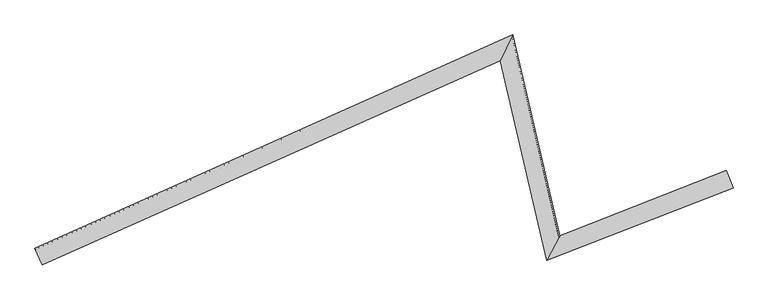
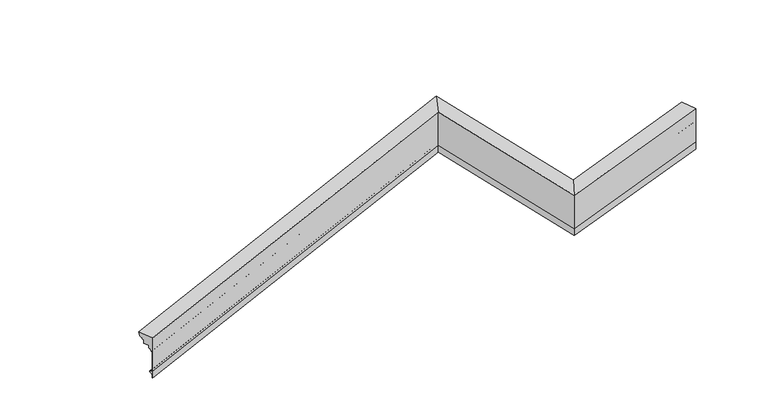
"""IFC4 building model written with IfcOpenShell, lengths in millimetres: proxy geometry, 41_GMA_lijst_1 : 41_GMA_lijst_1."""

from ifc_helpers import new_model, si_unit, frame, origin, place, context, project, spatial, polyline, circle_curve, ellipse_curve, source, transform, mapped, element, save
from ifc_brep_helpers import plane_surface, cylinder_surface, revolved_surface, advanced_brep


def generic_models_faa5d878(model_context):
    return source(origin(), model_context, "Body", "AdvancedBrep", [
        advanced_brep(
        [(-320.0822869, -45.7176461, 0.0), (-315.9983768, -54.845717, 0.0), (-315.9983768, -54.845717, 90.0), (-315.9983768, -54.845717, 546.0073397), (-396.3926245, 124.8458983, 546.0073397), (-392.3087144, 115.7178274, 528.6868317), (-376.232998, 79.7865073, 483.4042569), (-369.0135968, 63.6502052, 465.7265873), (-369.0135968, 63.6502052, 415.7265873), (-340.4262264, -0.2462912, 415.7265873), (-340.4262264, -0.2462912, 395.7265873), (-333.4250381, -15.8948591, 385.4258258), (-332.2538209, -18.5126823, 381.3300656), (-327.7077697, -28.6736987, 365.4324729), (-327.0543832, -30.1341027, 350.2103996), (-322.09322, -41.2229486, 353.9244378), (-320.0822869, -45.7176461, 353.0561969), (-320.0822869, -45.7176461, 88.0561969), (-332.0338853, -19.0042668, 82.3676402), (-332.0797901, -18.9016636, 62.47191), (-321.0256577, -43.6090895, 37.0771565), (-320.0822869, -45.7176461, 36.0), (4610.6792348, 2160.3110669, 0.0), (4603.6865732, 2146.2273243, 0.0), (4603.6865732, 2146.2273243, 90.0), (4603.6865732, 2146.2273243, 546.0073397), (4741.3413597, 2423.4743432, 546.0073397), (4734.3486981, 2409.3906006, 528.6868317), (4706.8231055, 2353.9520018, 483.4042569), (4694.4617095, 2329.0552271, 465.7265873), (4694.4617095, 2329.0552271, 415.7265873), (4645.5130785, 2230.4690292, 415.7265873), (4645.5130785, 2230.4690292, 395.7265873), (4633.5253168, 2206.324782, 385.4258258), (4631.5199038, 2202.2857305, 381.3300656), (4623.7359427, 2186.6082516, 365.4324729), (4622.6171837, 2184.3549875, 350.2103996), (4614.1224484, 2167.2459563, 353.9244378), (4610.6792348, 2160.3110669, 353.0561969), (4610.6792348, 2160.3110669, 88.0561969), (4631.1433199, 2201.5272625, 82.3676402), (4631.2219203, 2201.6855695, 62.47191), (4612.2945183, 2163.5643686, 37.0771565), (4610.6792348, 2160.3110669, 36.0), (5110.9375858, 8.3430809, 0.0), (5103.8132021, -5.1740306, 0.0), (5103.8132021, -5.1740306, 90.0), (5103.8132021, -5.1740306, 546.0073397), (5244.0610196, 260.9185125, 546.0073397), (5236.9366358, 247.401401, 528.6868317), (5208.8925381, 194.1932626, 483.4042569), (5196.298288, 170.2981595, 465.7265873), (5196.298288, 170.2981595, 415.7265873), (5146.4276017, 75.6783788, 415.7265873), (5146.4276017, 75.6783788, 395.7265873), (5134.2140241, 52.5055268, 385.4258258), (5132.1708348, 48.6289785, 381.3300656), (5124.2402456, 33.5822514, 365.4324729), (5123.1004124, 31.4196428, 350.2103996), (5114.44566, 14.998959, 353.9244378), (5110.9375858, 8.3430809, 353.0561969), (5110.9375858, 8.3430809, 88.0561969), (5131.7871571, 47.9010259, 82.3676402), (5131.8672381, 48.0529637, 62.47191), (5112.5832968, 11.4654925, 37.0771565), (5110.9375858, 8.3430809, 36.0), (7104.8613846, 786.9017358, 0.0), (7104.8613846, 786.9017358, 36.0), (7104.0211985, 789.0534902, 37.0771565), (7094.1761535, 814.2670942, 62.47191), (7094.2170373, 814.1623889, 82.3676402), (7104.8613846, 786.9017358, 88.0561969), (7104.8613846, 786.9017358, 353.0561969), (7103.0704048, 791.4885157, 353.9244378), (7098.6518876, 802.8045374, 350.2103996), (7098.0699677, 804.2948606, 365.4324729), (7094.021158, 814.6640445, 381.3300656), (7092.978047, 817.3354987, 385.4258258), (7086.7426401, 833.3046569, 395.7265873), (7086.7426401, 833.3046569, 415.7265873), (7061.2821211, 898.5101933, 415.7265873), (7061.2821211, 898.5101933, 465.7265873), (7054.8523691, 914.9770779, 483.4042569), (7040.5349948, 951.6445187, 528.6868317), (7036.8977778, 960.9595953, 546.0073397), (7108.4986016, 777.5866592, 546.0073397), (7108.4986016, 777.5866592, 90.0), (7108.4986016, 777.5866592, 0.0)],
        [
            (0, 1),
            (1, 2),
            (2, 3),
            (3, 4),
            (4, 5, circle_curve(frame((-398.3045101, 129.1192117, 531.7574646), z_axis=(0.9128070918396476, 0.4083910051497771, 0.0), x_axis=(-0.4083910051497771, 0.9128070918396476, 0.0)), 14.9991818)),
            (5, 6, circle_curve(frame((-377.2557163, 82.0724159, 520.9777245), z_axis=(-0.9128070918396476, -0.4083910051497771, 0.0), x_axis=(-0.4083910051497771, 0.9128070918396476, 0.0)), 37.6568294)),
            (6, 7, circle_curve(frame((-369.0135968, 63.6502052, 483.4042569), z_axis=(-0.9128070918396476, -0.4083910051497771, 0.0), x_axis=(-0.4083910051497771, 0.9128070918396476, 0.0)), 17.6776695)),
            (7, 8),
            (8, 9),
            (9, 10),
            (10, 11, circle_curve(frame((-335.6789229, -10.8571329, 395.6568101), z_axis=(-0.9128070918396477, -0.4083910051497771, 0.0), x_axis=(-0.33453432673767486, 0.747727795321934, -0.5735764363510506)), 11.624617)),
            (11, 12, circle_curve(frame((-336.1630624, -9.7750183, 377.679405), z_axis=(0.9128070918396477, 0.4083910051497771, 0.0), x_axis=(-0.33453432673767486, 0.747727795321934, -0.5735764363510506)), 10.2448165)),
            (12, 13, circle_curve(frame((-317.080196, -52.4277103, 395.5000152), z_axis=(-0.9128070918396477, -0.4083910051497771, 0.0), x_axis=(-0.33453432673767486, 0.747727795321934, -0.5735764363510506)), 39.7650034)),
            (13, 14, circle_curve(frame((-341.117916, 1.2997249, 354.2860988), z_axis=(0.9128070918396477, 0.4083910051497771, 0.0), x_axis=(-0.33453432673767486, 0.747727795321934, -0.5735764363510506)), 34.6767905)),
            (14, 15, circle_curve(frame((-325.357267, -33.9273784, 358.3422875), z_axis=(-0.9128070918396477, -0.4083910051497771, 0.0), x_axis=(-0.33453432673767486, 0.747727795321934, -0.5735764363510506)), 9.1321817)),
            (15, 16, circle_curve(frame((-321.331163, -42.9262453, 350.1101153), z_axis=(0.9128070918396476, 0.4083910051497771, 0.0), x_axis=(-0.4083910051497771, 0.9128070918396476, 0.0)), 4.2462933)),
            (16, 17),
            (17, 18),
            (18, 19, circle_curve(frame((-328.2882163, -27.376325, 72.3676402), z_axis=(-0.9128070918396476, -0.4083910051497771, 0.0), x_axis=(-0.4083910051497771, 0.9128070918396476, 0.0)), 13.5691339)),
            (19, 20, circle_curve(frame((-339.7944325, -1.658433, 15.2146431), z_axis=(0.9128070918396476, 0.4083910051497771, 0.0), x_axis=(-0.4083910051497771, 0.9128070918396476, 0.0)), 50.8929659)),
            (20, 21),
            (21, 0),
            (0, 22),
            (22, 23),
            (23, 1),
            (23, 24),
            (24, 2),
            (24, 25),
            (25, 3),
            (25, 26),
            (26, 4),
            (26, 27, ellipse_curve(frame((4744.6149796, 2430.0676581, 531.7574646), z_axis=(0.8956755111993515, -0.4447081949298666, 0.0), x_axis=(0.44470819492986674, 0.8956755111993515, 0.0)), 23.5849493, 14.9991818)),
            (27, 5),
            (27, 28, ellipse_curve(frame((4708.5742516, 2357.4789406, 520.9777245), z_axis=(-0.8956755111993515, 0.4447081949298666, 0.0), x_axis=(-0.44470819492986674, -0.8956755111993515, 0.0)), 59.2121906, 37.6568294)),
            (28, 6),
            (28, 29, ellipse_curve(frame((4694.4617095, 2329.0552271, 483.4042569), z_axis=(-0.8956755111993515, 0.4447081949298666, 0.0), x_axis=(-0.44470819492986674, -0.8956755111993515, 0.0)), 27.7966455, 17.6776695)),
            (29, 7),
            (29, 30),
            (30, 8),
            (30, 31),
            (31, 9),
            (31, 32),
            (32, 10),
            (32, 33, ellipse_curve(frame((4637.3845236, 2214.0975127, 395.6568101), z_axis=(-0.8956755111993516, 0.4447081949298666, 0.0), x_axis=(-0.4447081949298666, -0.8956755111993516, 0.0)), 18.2787306, 11.624617)),
            (33, 11),
            (33, 34, ellipse_curve(frame((4638.2134898, 2215.7671125, 377.679405), z_axis=(0.8956755111993516, -0.4447081949298666, 0.0), x_axis=(0.4447081949298666, 0.8956755111993516, 0.0)), 16.1091105, 10.2448165)),
            (34, 12),
            (34, 35, ellipse_curve(frame((4605.5389144, 2149.9580779, 395.5000152), z_axis=(-0.8956755111993516, 0.4447081949298666, 0.0), x_axis=(-0.4447081949298666, -0.8956755111993516, 0.0)), 62.5271165, 39.7650034)),
            (35, 13),
            (35, 36, ellipse_curve(frame((4646.6974216, 2232.8543846, 354.2860988), z_axis=(0.8956755111993516, -0.4447081949298666, 0.0), x_axis=(0.4447081949298666, 0.8956755111993516, 0.0)), 54.5263306, 34.6767905)),
            (36, 14),
            (36, 37, ellipse_curve(frame((4619.7113022, 2178.5023251, 358.3422875), z_axis=(-0.8956755111993516, 0.4447081949298666, 0.0), x_axis=(-0.4447081949298666, -0.8956755111993516, 0.0)), 14.3595861, 9.1321817)),
            (37, 15),
            (37, 38, ellipse_curve(frame((4612.8176188, 2164.617932, 350.1101153), z_axis=(0.8956755111993515, -0.4447081949298666, 0.0), x_axis=(0.44470819492986674, 0.8956755111993515, 0.0)), 6.6769384, 4.2462933)),
            (38, 16),
            (38, 39),
            (39, 17),
            (39, 40),
            (40, 18),
            (40, 41, ellipse_curve(frame((4624.7298104, 2188.6099754, 72.3676402), z_axis=(-0.8956755111993515, 0.4447081949298666, 0.0), x_axis=(-0.44470819492986674, -0.8956755111993515, 0.0)), 21.3363195, 13.5691339)),
            (41, 19),
            (41, 42, ellipse_curve(frame((4644.4312914, 2228.2902292, 15.2146431), z_axis=(0.8956755111993515, -0.4447081949298666, 0.0), x_axis=(0.44470819492986674, 0.8956755111993515, 0.0)), 80.0248998, 50.8929659)),
            (42, 20),
            (42, 43),
            (43, 21),
            (43, 22),
            (22, 44),
            (44, 45),
            (45, 23),
            (45, 46),
            (46, 24),
            (46, 47),
            (47, 25),
            (47, 48),
            (48, 26),
            (48, 49, ellipse_curve(frame((5247.3963053, 267.2465587, 531.7574646), z_axis=(0.8846452460143381, -0.46626471955771137, 0.0), x_axis=(-0.46626471955771137, -0.8846452460143381, 0.0)), 22.9182957, 14.9991818)),
            (49, 27),
            (49, 50, ellipse_curve(frame((5210.6766708, 197.5783022, 520.9777245), z_axis=(-0.8846452460143381, 0.46626471955771137, 0.0), x_axis=(0.46626471955771137, 0.8846452460143381, 0.0)), 57.5384952, 37.6568294)),
            (50, 28),
            (50, 51, ellipse_curve(frame((5196.298288, 170.2981595, 483.4042569), z_axis=(-0.8846452460143381, 0.46626471955771137, 0.0), x_axis=(0.46626471955771137, 0.8846452460143381, 0.0)), 27.0109438, 17.6776695)),
            (51, 29),
            (51, 52),
            (52, 30),
            (52, 53),
            (53, 31),
            (53, 54),
            (54, 32),
            (54, 55, ellipse_curve(frame((5138.1459276, 59.9655374, 395.6568101), z_axis=(-0.8846452460143381, 0.46626471955771137, 0.0), x_axis=(0.46626471955771137, 0.8846452460143381, 0.0)), 17.7620629, 11.624617)),
            (55, 33),
            (55, 56, ellipse_curve(frame((5138.9905092, 61.5679641, 377.679405), z_axis=(0.8846452460143381, -0.46626471955771137, 0.0), x_axis=(-0.46626471955771137, -0.8846452460143381, 0.0)), 15.6537694, 10.2448165)),
            (56, 34),
            (56, 57, ellipse_curve(frame((5105.7004362, -1.5933764, 395.5000152), z_axis=(-0.8846452460143381, 0.46626471955771137, 0.0), x_axis=(0.46626471955771137, 0.8846452460143381, 0.0)), 60.7597213, 39.7650034)),
            (57, 35),
            (57, 58, ellipse_curve(frame((5147.6342545, 77.9677643, 354.2860988), z_axis=(0.8846452460143381, -0.46626471955771137, 0.0), x_axis=(-0.46626471955771137, -0.8846452460143381, 0.0)), 52.985086, 34.6767905)),
            (58, 36),
            (58, 59, ellipse_curve(frame((5120.1397922, 25.8024505, 358.3422875), z_axis=(-0.8846452460143381, 0.46626471955771137, 0.0), x_axis=(0.46626471955771137, 0.8846452460143381, 0.0)), 13.9536972, 9.1321817)),
            (59, 37),
            (59, 60, ellipse_curve(frame((5113.116251, 12.476668, 350.1101153), z_axis=(0.8846452460143381, -0.46626471955771137, 0.0), x_axis=(-0.46626471955771137, -0.8846452460143381, 0.0)), 6.4882076, 4.2462933)),
            (60, 38),
            (60, 61),
            (61, 39),
            (61, 62),
            (62, 40),
            (62, 63, ellipse_curve(frame((5125.252835, 35.5034398, 72.3676402), z_axis=(-0.8846452460143381, 0.46626471955771137, 0.0), x_axis=(0.46626471955771137, 0.8846452460143381, 0.0)), 20.7332258, 13.5691339)),
            (63, 41),
            (63, 64, ellipse_curve(frame((5145.3254368, 73.5872385, 15.2146431), z_axis=(0.8846452460143381, -0.46626471955771137, 0.0), x_axis=(-0.46626471955771137, -0.8846452460143381, 0.0)), 77.7629111, 50.8929659)),
            (64, 42),
            (64, 65),
            (65, 43),
            (65, 44),
            (66, 67),
            (67, 68),
            (68, 69, circle_curve(frame((7087.3053292, 831.8635848, 15.2146431), z_axis=(-0.9315076625045138, -0.3637216995112841, 0.0), x_axis=(-0.3637216995112841, 0.9315076625045138, 0.0)), 50.8929659)),
            (69, 70, circle_curve(frame((7097.5530097, 805.6188134, 72.3676402), z_axis=(0.9315076625045138, 0.3637216995112841, 0.0), x_axis=(-0.3637216995112841, 0.9315076625045138, 0.0)), 13.5691339)),
            (70, 71),
            (71, 72),
            (72, 73, circle_curve(frame((7103.749109, 789.7503237, 350.1101153), z_axis=(-0.9315076625045138, -0.3637216995112841, 0.0), x_axis=(-0.3637216995112841, 0.9315076625045138, 0.0)), 4.2462933)),
            (73, 74, circle_curve(frame((7100.1633753, 798.9335494, 358.3422875), z_axis=(0.9315076625045138, 0.3637216995112842, 0.0), x_axis=(-0.2979433737069339, 0.7630464060114299, -0.5735764363510502)), 9.1321817)),
            (74, 75, circle_curve(frame((7086.1266067, 834.8823461, 354.2860988), z_axis=(-0.9315076625045138, -0.3637216995112842, 0.0), x_axis=(-0.2979433737069339, 0.7630464060114299, -0.5735764363510502)), 34.6767905)),
            (75, 76, circle_curve(frame((7107.5351105, 780.0542033, 395.5000152), z_axis=(0.9315076625045138, 0.3637216995112842, 0.0), x_axis=(-0.2979433737069339, 0.7630464060114299, -0.5735764363510502)), 39.7650034)),
            (76, 77, circle_curve(frame((7090.5395045, 823.580716, 377.679405), z_axis=(-0.9315076625045138, -0.3637216995112842, 0.0), x_axis=(-0.2979433737069339, 0.7630464060114299, -0.5735764363510502)), 10.2448165)),
            (77, 78, circle_curve(frame((7090.9706894, 822.4764322, 395.6568101), z_axis=(0.9315076625045138, 0.3637216995112842, 0.0), x_axis=(-0.2979433737069339, 0.7630464060114299, -0.5735764363510502)), 11.624617)),
            (78, 79),
            (79, 80),
            (80, 81),
            (81, 82, circle_curve(frame((7061.2821211, 898.5101933, 483.4042569), z_axis=(0.9315076625045138, 0.3637216995112841, 0.0), x_axis=(-0.3637216995112841, 0.9315076625045138, 0.0)), 17.6776695)),
            (82, 83, circle_curve(frame((7053.9415145, 917.3098176, 520.9777245), z_axis=(0.9315076625045138, 0.3637216995112841, 0.0), x_axis=(-0.3637216995112841, 0.9315076625045138, 0.0)), 37.6568294)),
            (83, 84, circle_curve(frame((7035.1950119, 965.3204556, 531.7574646), z_axis=(-0.9315076625045138, -0.3637216995112841, 0.0), x_axis=(-0.3637216995112841, 0.9315076625045138, 0.0)), 14.9991818)),
            (84, 85),
            (85, 86),
            (86, 87),
            (87, 66),
            (44, 66),
            (87, 45),
            (86, 46),
            (85, 47),
            (84, 48),
            (83, 49),
            (82, 50),
            (81, 51),
            (80, 52),
            (79, 53),
            (78, 54),
            (77, 55),
            (76, 56),
            (75, 57),
            (74, 58),
            (73, 59),
            (72, 60),
            (71, 61),
            (70, 62),
            (69, 63),
            (68, 64),
            (67, 65),
        ],
        [
            plane_surface(frame((-315.9983768, -54.845717, 580.4104812), z_axis=(-0.9128070918396477, -0.40839100514977694, 0.0), x_axis=(0.40839100514977694, -0.9128070918396477, 0.0))),
            plane_surface(frame((-320.0822869, -45.7176461, 0.0), z_axis=(0.0, 0.0, -1.0), x_axis=(0.9128070918396477, 0.4083910051497769, 0.0))),
            plane_surface(frame((-315.9983768, -54.845717, 0.0), z_axis=(0.4083910051497769, -0.9128070918396477, 0.0), x_axis=(0.9128070918396477, 0.4083910051497769, 0.0))),
            plane_surface(frame((-315.9983768, -54.845717, 90.0), z_axis=(0.408391005149777, -0.9128070918396476, 0.0), x_axis=(0.9128070918396476, 0.408391005149777, 0.0))),
            plane_surface(frame((-315.9983768, -54.845717, 546.0073397), z_axis=(0.0, 0.0, 1.0000000000000002), x_axis=(0.9128070918396477, 0.40839100514977694, 0.0))),
            revolved_surface(polyline([(4755.103399845207, 2451.1921195884997, 531.7574646), (-404.4300410502379, 142.81057121055002, 531.7574646)]), (-398.3045101, 129.1192117, 531.7574646), (0.9128070918396476, 0.4083910051497771, 0.0)),
            cylinder_surface(frame((-377.2557163, 82.0724159, 520.9777245), z_axis=(-0.9128070918396476, -0.4083910051497771, 0.0), x_axis=(-0.4083910051497771, 0.9128070918396476, 0.0)), 37.6568294),
            cylinder_surface(frame((-369.0135968, 63.6502052, 483.4042569), z_axis=(-0.9128070918396476, -0.4083910051497771, 0.0), x_axis=(-0.4083910051497771, 0.9128070918396476, 0.0)), 17.6776695),
            plane_surface(frame((-369.0135968, 63.6502052, 465.7265873), z_axis=(-0.4083910051497768, 0.9128070918396477, 0.0), x_axis=(0.9128070918396477, 0.4083910051497768, 0.0))),
            plane_surface(frame((-369.0135968, 63.6502052, 415.7265873), z_axis=(0.0, 0.0, -1.0), x_axis=(0.9128070918396477, 0.4083910051497769, 0.0))),
            plane_surface(frame((-340.4262264, -0.2462912, 415.7265873), z_axis=(-0.4083910051497769, 0.9128070918396477, 0.0), x_axis=(0.9128070918396477, 0.4083910051497769, 0.0))),
            cylinder_surface(frame((-335.6789229, -10.8571329, 395.6568101), z_axis=(-0.9128070918396477, -0.4083910051497771, 0.0), x_axis=(-0.33453432673767486, 0.747727795321934, -0.5735764363510506)), 11.624617),
            revolved_surface(polyline([(4646.133991374211, 2228.5044411719005, 371.80321966085955), (-339.59030520745455, -2.11468425261706, 371.80321966085955)]), (-336.1630624, -9.7750183, 377.679405), (0.9128070918396477, 0.4083910051497771, 0.0)),
            cylinder_surface(frame((-317.080196, -52.4277103, 395.5000152), z_axis=(-0.9128070918396477, -0.4083910051497771, 0.0), x_axis=(-0.33453432673767486, 0.747727795321934, -0.5735764363510506)), 39.7650034),
            revolved_surface(polyline([(4673.506840214611, 2275.967863468368, 334.396308880918), (-352.71849276334086, 27.22852500940559, 334.396308880918)]), (-341.117916, 1.2997249, 354.2860988), (0.9128070918396477, 0.4083910051497771, 0.0)),
            cylinder_surface(frame((-325.357267, -33.9273784, 358.3422875), z_axis=(-0.9128070918396477, -0.4083910051497771, 0.0), x_axis=(-0.33453432673767486, 0.747727795321934, -0.5735764363510506)), 9.1321817),
            revolved_surface(polyline([(4615.786908049704, 2170.598302156147, 350.1101153), (-323.0653110049939, -39.05019866890786, 350.1101153)]), (-321.331163, -42.9262453, 350.1101153), (0.9128070918396476, 0.4083910051497771, 0.0)),
            plane_surface(frame((-320.0822869, -45.7176461, 353.0561969), z_axis=(-0.408391005149777, 0.9128070918396476, 0.0), x_axis=(0.9128070918396476, 0.408391005149777, 0.0))),
            plane_surface(frame((-320.0822869, -45.7176461, 88.0561969), z_axis=(-0.07792467741344727, 0.17417180416651107, 0.9816271834476635), x_axis=(0.9128070918396477, 0.4083910051497769, 0.0))),
            cylinder_surface(frame((-328.2882163, -27.376325, 72.3676402), z_axis=(-0.9128070918396476, -0.4083910051497771, 0.0), x_axis=(-0.4083910051497771, 0.9128070918396476, 0.0)), 13.5691339),
            revolved_surface(polyline([(4680.019020159113, 2299.9665721932106, 15.2146431), (-360.57866202829814, 44.797027185144906, 15.2146431)]), (-339.7944325, -1.658433, 15.2146431), (0.9128070918396476, 0.4083910051497771, 0.0)),
            plane_surface(frame((-321.0256577, -43.6090895, 37.0771565), z_axis=(-0.17259349670693577, 0.38576894645785487, -0.90630778703665), x_axis=(0.9128070918396477, 0.40839100514977694, 0.0))),
            plane_surface(frame((-320.0822869, -45.7176461, 36.0), z_axis=(-0.4083910051497769, 0.9128070918396477, 0.0), x_axis=(0.9128070918396477, 0.4083910051497769, 0.0))),
            plane_surface(frame((4610.6792348, 2160.3110669, 0.0), z_axis=(0.0, 0.0, -1.0000000000000002), x_axis=(0.2264279060198721, -0.9740279274104291, 0.0))),
            plane_surface(frame((4603.6865732, 2146.2273243, 0.0), z_axis=(-0.974027927410429, -0.2264279060198726, 0.0), x_axis=(0.2264279060198726, -0.974027927410429, 0.0))),
            plane_surface(frame((4603.6865732, 2146.2273243, 90.0), z_axis=(-0.974027927410429, -0.22642790601987234, 0.0), x_axis=(0.22642790601987234, -0.974027927410429, 0.0))),
            plane_surface(frame((4603.6865732, 2146.2273243, 546.0073397), z_axis=(0.0, 0.0, 1.0), x_axis=(0.22642790601987234, -0.974027927410429, 0.0))),
            revolved_surface(polyline([(5265.929556577451, 253.7644640328915, 531.7574646), (4755.103399867837, 2451.1921196295175, 531.7574646)]), (4799.9898007, 2191.8610557, 531.7574646), (0.22642790601987206, -0.9740279274104291, 0.0)),
            cylinder_surface(frame((4749.7876348, 2180.1907832, 520.9777245), z_axis=(-0.22642790601987206, 0.9740279274104291, 0.0), x_axis=(0.9740279274104291, 0.22642790601987206, 0.0)), 37.6568294),
            cylinder_surface(frame((4730.1298694, 2175.6210306, 483.4042569), z_axis=(-0.22642790601987206, 0.9740279274104291, 0.0), x_axis=(0.9740279274104291, 0.22642790601987206, 0.0)), 17.6776695),
            plane_surface(frame((4694.4617095, 2329.0552271, 465.7265873), z_axis=(0.974027927410429, 0.22642790601987225, 0.0), x_axis=(0.22642790601987225, -0.974027927410429, 0.0))),
            plane_surface(frame((4694.4617095, 2329.0552271, 415.7265873), z_axis=(0.0, 0.0, -1.0), x_axis=(0.22642790601987248, -0.974027927410429, 0.0))),
            plane_surface(frame((4645.5130785, 2230.4690292, 415.7265873), z_axis=(0.974027927410429, 0.22642790601987217, 0.0), x_axis=(0.22642790601987217, -0.974027927410429, 0.0))),
            cylinder_surface(frame((4650.6254168, 2157.1389869, 395.6568101), z_axis=(-0.22642790601987206, 0.974027927410429, 0.0), x_axis=(0.7978769679328198, 0.18547888210025315, -0.5735764363510504)), 11.624617),
            revolved_surface(polyline([(5149.844549294588, 51.93984087414674, 371.80321966085955), (4643.572709017159, 2229.776133051008, 371.80321966085955)]), (4651.7801076, 2157.4074127, 377.679405), (0.22642790601987206, -0.974027927410429, 0.0)),
            cylinder_surface(frame((4606.2667525, 2146.827127, 395.5000152), z_axis=(-0.22642790601987206, 0.974027927410429, 0.0), x_axis=(0.7978769679328198, 0.18547888210025315, -0.5735764363510504)), 39.7650034),
            revolved_surface(polyline([(5184.373153056153, 45.37836525271359, 334.396308880918), (4664.837377707266, 2280.27230290294, 334.396308880918)]), (4663.59762, 2160.1545768, 354.2860988), (0.22642790601987206, -0.974027927410429, 0.0)),
            cylinder_surface(frame((4626.0078787, 2151.4162582, 358.3422875), z_axis=(-0.22642790601987206, 0.974027927410429, 0.0), x_axis=(0.7978769679328198, 0.18547888210025315, -0.5735764363510504)), 9.1321817),
            revolved_surface(polyline([(5118.363045238202, 8.659864594568717, 350.1101153), (4615.786907948484, 2170.598302197223, 350.1101153)]), (4616.405469, 2149.184029, 350.1101153), (0.22642790601987206, -0.9740279274104291, 0.0)),
            plane_surface(frame((4610.6792348, 2160.3110669, 353.0561969), z_axis=(0.974027927410429, 0.22642790601987253, 0.0), x_axis=(0.22642790601987253, -0.974027927410429, 0.0))),
            plane_surface(frame((4610.6792348, 2160.3110669, 88.0561969), z_axis=(0.18585329029788442, 0.04320448127286722, 0.9816271834476636), x_axis=(0.2264279060198721, -0.9740279274104291, 0.0))),
            cylinder_surface(frame((4632.9983031, 2153.0412908, 72.3676402), z_axis=(-0.22642790601987206, 0.9740279274104291, 0.0), x_axis=(0.9740279274104291, 0.22642790601987206, 0.0)), 13.5691339),
            revolved_surface(polyline([(5208.209674997979, 27.841824265728064, 15.2146431), (4680.019020071599, 2299.9665722212567, 15.2146431)]), (4660.4410621, 2159.420786, 15.2146431), (0.22642790601987206, -0.9740279274104291, 0.0)),
            plane_surface(frame((4612.2945183, 2163.5643686, 37.0771565), z_axis=(0.41164198956909176, 0.09569256805170483, -0.90630778703665), x_axis=(0.22642790601987253, -0.974027927410429, 0.0))),
            plane_surface(frame((4610.6792348, 2160.3110669, 36.0), z_axis=(0.9740279274104291, 0.2264279060198721, 0.0), x_axis=(0.2264279060198721, -0.9740279274104291, 0.0))),
            plane_surface(frame((7108.4986016, 777.5866592, 580.4104812), z_axis=(0.9315076625045137, 0.36372169951128447, 0.0), x_axis=(0.36372169951128447, -0.9315076625045137, 0.0))),
            plane_surface(frame((5110.9375858, 8.3430809, 0.0), z_axis=(0.0, 0.0, -1.0), x_axis=(0.9315076625045137, 0.3637216995112846, 0.0))),
            plane_surface(frame((5103.8132021, -5.1740306, 0.0), z_axis=(0.3637216995112847, -0.9315076625045136, 0.0), x_axis=(0.9315076625045136, 0.3637216995112847, 0.0))),
            plane_surface(frame((5103.8132021, -5.1740306, 90.0), z_axis=(0.3637216995112847, -0.9315076625045136, 0.0), x_axis=(0.9315076625045136, 0.3637216995112847, 0.0))),
            plane_surface(frame((5103.8132021, -5.1740306, 546.0073397), z_axis=(0.0, 0.0, 1.0), x_axis=(0.9315076625045136, 0.3637216995112847, 0.0))),
            revolved_surface(polyline([(7029.739483991484, 979.2923084111399, 531.7574646), (5225.799256772772, 274.9157029663272, 531.7574646)]), (5030.5096124, 182.5597658, 531.7574646), (0.9315076625045138, 0.3637216995112841, 0.0)),
            cylinder_surface(frame((5049.256115, 134.5491278, 520.9777245), z_axis=(-0.9315076625045138, -0.3637216995112841, 0.0), x_axis=(-0.3637216995112841, 0.9315076625045138, 0.0)), 37.6568294),
            cylinder_surface(frame((5056.5967217, 115.7495035, 483.4042569), z_axis=(-0.9315076625045138, -0.3637216995112841, 0.0), x_axis=(-0.3637216995112841, 0.9315076625045138, 0.0)), 17.6776695),
            plane_surface(frame((5196.298288, 170.2981595, 465.7265873), z_axis=(-0.3637216995112847, 0.9315076625045136, 0.0), x_axis=(0.9315076625045136, 0.3637216995112847, 0.0))),
            plane_surface(frame((5196.298288, 170.2981595, 415.7265873), z_axis=(0.0, 0.0, -1.0), x_axis=(0.9315076625045137, 0.36372169951128447, 0.0))),
            plane_surface(frame((5146.4276017, 75.6783788, 415.7265873), z_axis=(-0.3637216995112846, 0.9315076625045137, 0.0), x_axis=(0.9315076625045137, 0.3637216995112846, 0.0))),
            cylinder_surface(frame((5086.2852899, 39.7157423, 395.6568101), z_axis=(-0.9315076625045138, -0.3637216995112842, 0.0), x_axis=(-0.2979433737069339, 0.7630464060114299, -0.5735764363510502)), 11.624617),
            revolved_surface(polyline([(7087.487129310641, 831.3979864103678, 371.80321966085955), (5124.913071527164, 65.08032693507124, 371.80321966085955)]), (5085.8541051, 40.8200262, 377.679405), (0.9315076625045138, 0.3637216995112842, 0.0)),
            cylinder_surface(frame((5102.849711, -2.7064866, 395.5000152), z_axis=(-0.9315076625045138, -0.3637216995112842, 0.0), x_axis=(-0.2979433737069339, 0.7630464060114299, -0.5735764363510502)), 39.7650034),
            revolved_surface(polyline([(7075.794886821788, 861.3423464905661, 334.396308880918), (5099.984757128476, 89.85645623877255, 334.396308880918)]), (5081.4412073, 52.1216563, 354.2860988), (0.9315076625045138, 0.3637216995112842, 0.0)),
            cylinder_surface(frame((5095.4779758, 16.1728595, 358.3422875), z_axis=(-0.9315076625045138, -0.3637216995112842, 0.0), x_axis=(-0.2979433737069339, 0.7630464060114299, -0.5735764363510502)), 9.1321817),
            revolved_surface(polyline([(7102.204639982559, 793.7057784837059, 350.1101153), (5107.002090684343, 14.647815451139888, 350.1101153)]), (5099.0637095, 6.9896339, 350.1101153), (0.9315076625045138, 0.3637216995112841, 0.0)),
            plane_surface(frame((5110.9375858, 8.3430809, 353.0561969), z_axis=(-0.36372169951128447, 0.9315076625045137, 0.0), x_axis=(0.9315076625045137, 0.36372169951128447, 0.0))),
            plane_surface(frame((5110.9375858, 8.3430809, 88.0561969), z_axis=(-0.06940137208039829, 0.17774004126804208, 0.9816271834476635), x_axis=(0.9315076625045137, 0.3637216995112846, 0.0))),
            cylinder_surface(frame((5092.8676102, 22.8581235, 72.3676402), z_axis=(-0.9315076625045138, -0.3637216995112841, 0.0), x_axis=(-0.3637216995112841, 0.9315076625045138, 0.0)), 13.5691339),
            revolved_surface(polyline([(7068.794453152303, 879.2707725426488, 15.2146431), (5072.045582753289, 99.60902431172994, 15.2146431)]), (5082.6199297, 49.102895, 15.2146431), (0.9315076625045138, 0.3637216995112841, 0.0)),
            plane_surface(frame((5112.5832968, 11.4654925, 37.0771565), z_axis=(-0.15371543240483235, 0.3936721491257996, -0.90630778703665), x_axis=(0.9315076625045136, 0.3637216995112846, 0.0))),
            plane_surface(frame((5110.9375858, 8.3430809, 36.0), z_axis=(-0.36372169951128447, 0.9315076625045137, 0.0), x_axis=(0.9315076625045137, 0.36372169951128447, 0.0))),
        ],
        [
            (0, [[1, 2, 3, 4, 5, 6, 7, 8, 9, 10, 11, 12, 13, 14, 15, 16, 17, 18, 19, 20, 21, 22]]),
            (1, [[-1, 23, 24, 25]]),
            (2, [[-2, -25, 26, 27]]),
            (3, [[-3, -27, 28, 29]]),
            (4, [[-4, -29, 30, 31]]),
            (5, [[-5, -31, 32, 33]]),
            (6, [[-6, -33, 34, 35]]),
            (7, [[-7, -35, 36, 37]]),
            (8, [[-8, -37, 38, 39]]),
            (9, [[-9, -39, 40, 41]]),
            (10, [[-10, -41, 42, 43]]),
            (11, [[-11, -43, 44, 45]]),
            (12, [[-12, -45, 46, 47]]),
            (13, [[-13, -47, 48, 49]]),
            (14, [[-14, -49, 50, 51]]),
            (15, [[-15, -51, 52, 53]]),
            (16, [[-16, -53, 54, 55]]),
            (17, [[-17, -55, 56, 57]]),
            (18, [[-18, -57, 58, 59]]),
            (19, [[-19, -59, 60, 61]]),
            (20, [[-20, -61, 62, 63]]),
            (21, [[-21, -63, 64, 65]]),
            (22, [[-22, -65, 66, -23]]),
            (23, [[-24, 67, 68, 69]]),
            (24, [[-26, -69, 70, 71]]),
            (25, [[-28, -71, 72, 73]]),
            (26, [[-30, -73, 74, 75]]),
            (27, [[-32, -75, 76, 77]]),
            (28, [[-34, -77, 78, 79]]),
            (29, [[-36, -79, 80, 81]]),
            (30, [[-38, -81, 82, 83]]),
            (31, [[-40, -83, 84, 85]]),
            (32, [[-42, -85, 86, 87]]),
            (33, [[-44, -87, 88, 89]]),
            (34, [[-46, -89, 90, 91]]),
            (35, [[-48, -91, 92, 93]]),
            (36, [[-50, -93, 94, 95]]),
            (37, [[-52, -95, 96, 97]]),
            (38, [[-54, -97, 98, 99]]),
            (39, [[-56, -99, 100, 101]]),
            (40, [[-58, -101, 102, 103]]),
            (41, [[-60, -103, 104, 105]]),
            (42, [[-62, -105, 106, 107]]),
            (43, [[-64, -107, 108, 109]]),
            (44, [[-66, -109, 110, -67]]),
            (45, [[111, 112, 113, 114, 115, 116, 117, 118, 119, 120, 121, 122, 123, 124, 125, 126, 127, 128, 129, 130, 131, 132]]),
            (46, [[-68, 133, -132, 134]]),
            (47, [[-70, -134, -131, 135]]),
            (48, [[-72, -135, -130, 136]]),
            (49, [[-74, -136, -129, 137]]),
            (50, [[-76, -137, -128, 138]]),
            (51, [[-78, -138, -127, 139]]),
            (52, [[-80, -139, -126, 140]]),
            (53, [[-82, -140, -125, 141]]),
            (54, [[-84, -141, -124, 142]]),
            (55, [[-86, -142, -123, 143]]),
            (56, [[-88, -143, -122, 144]]),
            (57, [[-90, -144, -121, 145]]),
            (58, [[-92, -145, -120, 146]]),
            (59, [[-94, -146, -119, 147]]),
            (60, [[-96, -147, -118, 148]]),
            (61, [[-98, -148, -117, 149]]),
            (62, [[-100, -149, -116, 150]]),
            (63, [[-102, -150, -115, 151]]),
            (64, [[-104, -151, -114, 152]]),
            (65, [[-106, -152, -113, 153]]),
            (66, [[-108, -153, -112, 154]]),
            (67, [[-110, -154, -111, -133]]),
        ],
    ),
    ])


if __name__ == "__main__":
    model = new_model("IFC4")
    model_context = context("Model", 3, world=origin())
    ifc_project = project(units=[si_unit("LENGTHUNIT", "METRE", prefix="MILLI")], contexts=[model_context])
    site = spatial("IfcSite", under=ifc_project)
    building = spatial("IfcBuilding", under=site)
    placement = place(None, origin())
    generic_models_shape = generic_models_faa5d878(model_context)
    element("IfcBuildingElementProxy", 1, Name="41_GMA_lijst_1 : 41_GMA_lijst_1", ObjectType="41_GMA_lijst_1 : 41_GMA_lijst_1", at=placement, inside=building, context=model_context, shape_type="MappedRepresentation", body=[
        mapped(generic_models_shape, transform((0.0, 0.0, 0.0), x_axis=(1.0, 0.0, 0.0), y_axis=(0.0, 1.0, 0.0), z_axis=(0.0, 0.0, 1.0))),
    ])
    save(model, "model.ifc")

# Revit data of these elements
# Type "41_GMA_lijst_1 : 41_GMA_lijst_1"
#   Default Elevation = 0
